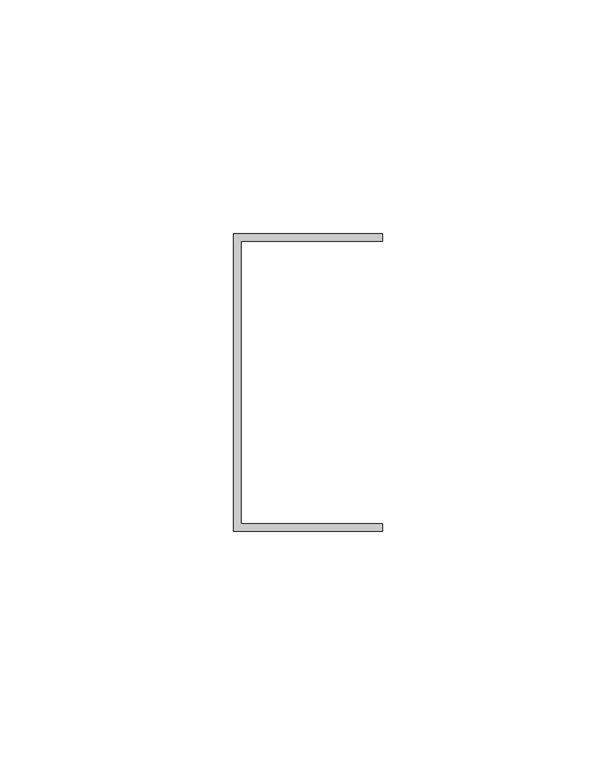
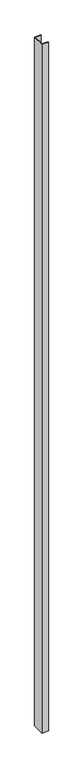
"""IFC4 building model written with IfcOpenShell, lengths in millimetres: proxy geometry, Generic Models 7:Generic Models 1:3:Generic Models 1:3 : Generic Models 7:Generic Models 1:305549:3:Generic Models 1:3:Generic Models 1:3 : Generic Models 7:Generic Models 1:305549:3 : Generic Models 7:Generic Models 1:3:Generic Models 1:3 : Generic Models 7:Generic Models 1:305549:301244:30 : Generic Models 7:Generic Models 1:3:Generic Models 1:3 : Generic Models 7:Generic Models 1:305549:3:Generic Models 1:3:Generic Models 1:3 : Generic Models 7:Generic Models 1:305549:3 : Generic Models 7:Generic Models 1:3:Generic Models 1:3 : Generic Models 7:Generic Models 1:305549:301244:308848."""

from ifc_helpers import new_model, si_unit, frame, origin, place, context, project, spatial, polyline, outline, extrude, source, transform, mapped, element, save


def generic_models_0b7faaaa(model_context):
    return source(origin(), model_context, "Body", "SweptSolid", [
        extrude(outline(polyline([(593738.0867239, -579013.3913841), (593769.8367239, -579013.3913841), (593769.8367239, -579014.9788841), (593739.6742239, -579014.9788841), (593739.6742239, -579075.3038841), (593769.8367239, -579075.3038841), (593769.8367239, -579076.8913841), (593738.0867239, -579076.8913841), (593738.0867239, -579013.3913841)])), frame((0.0, 0.0, 38.1), z_axis=(0.0, 0.0, 1.0), x_axis=(1.0, 0.0, 0.0)), (0.0, 0.0, 1.0), 3657.6),
    ])


if __name__ == "__main__":
    model = new_model("IFC4")
    model_context = context("Model", 3, world=origin())
    ifc_project = project(units=[si_unit("LENGTHUNIT", "METRE", prefix="MILLI")], contexts=[model_context])
    site = spatial("IfcSite", under=ifc_project)
    building = spatial("IfcBuilding", under=site)
    placement = place(None, origin())
    generic_models_shape = generic_models_0b7faaaa(model_context)
    element("IfcBuildingElementProxy", 1, Name="Generic Models 7:Generic Models 1:3:Generic Models 1:3 : Generic Models 7:Generic Models 1:305549:3:Generic Models 1:3:Generic Models 1:3 : Generic Models 7:Generic Models 1:305549:3 : Generic Models 7:Generic Models 1:3:Generic Models 1:3 : Generic Models 7:Generic Models 1:305549:301244:30 : Generic Models 7:Generic Models 1:3:Generic Models 1:3 : Generic Models 7:Generic Models 1:305549:3:Generic Models 1:3:Generic Models 1:3 : Generic Models 7:Generic Models 1:305549:3 : Generic Models 7:Generic Models 1:3:Generic Models 1:3 : Generic Models 7:Generic Models 1:305549:301244:308848", ObjectType="Generic Models 7:Generic Models 1:3:Generic Models 1:3 : Generic Models 7:Generic Models 1:305549:3:Generic Models 1:3:Generic Models 1:3 : Generic Models 7:Generic Models 1:305549:3 : Generic Models 7:Generic Models 1:3:Generic Models 1:3 : Generic Models 7:Generic Models 1:305549:301244:30 : Generic Models 7:Generic Models 1:3:Generic Models 1:3 : Generic Models 7:Generic Models 1:305549:3:Generic Models 1:3:Generic Models 1:3 : Generic Models 7:Generic Models 1:305549:3 : Generic Models 7:Generic Models 1:3:Generic Models 1:3 : Generic Models 7:Generic Models 1:305549:301244:308848", at=placement, inside=building, context=model_context, shape_type="MappedRepresentation", body=[
        mapped(generic_models_shape, transform((0.0, 0.0, 0.0), x_axis=(1.0, 0.0, 0.0), y_axis=(0.0, 1.0, 0.0), z_axis=(0.0, 0.0, 1.0))),
    ])
    save(model, "model.ifc")

# Revit data of these elements
# Type "Generic Models 7:Generic Models 1:3:Generic Models 1:3 : Generic Models 7:Generic Models 1:305549:3:Generic Models 1:3:Generic Models 1:3 : Generic Models 7:Generic Models 1:305549:3 : Generic Models 7:Generic Models 1:3:Generic Models 1:3 : Generic Models 7:Generic Models 1:305549:301244:30 : Generic Models 7:Generic Models 1:3:Generic Models 1:3 : Generic Models 7:Generic Models 1:305549:3:Generic Models 1:3:Generic Models 1:3 : Generic Models 7:Generic Models 1:305549:3 : Generic Models 7:Generic Models 1:3:Generic Models 1:3 : Generic Models 7:Generic Models 1:305549:301244:308848"
#   NameOverride = "Generic Models 7:Generic Models 1:3:Generic Models 1:3 : Generic Models 7:Generic Models 1:305549:3:Generic Models 1:3:Generic Models 1:3 : Generic Models 7:Generic Models 1:305549:3 : Generic Models 7:Generic Models 1:3:Generic Models 1:3 : Generic Models 7:Generic Models 1:305549:301244:308848"
#   ObjectTypeOverride = "Generic Models 1:3:Generic Models 1:3 : Generic Models 7:Generic Models 1:305549:3 : Generic Models 7:Generic Models 1:3:Generic Models 1:3 : Generic Models 7:Generic Models 1:305549:301244"
#   Reference = "Generic Models 1"
#   Tag = "308848"
# Element 1 (IfcBuildingElementProxy, "Generic Models 7:Generic Models 1:3:Generic Models 1:3 : Generic Models 7:Generic Models 1:305549:3:Generic Models 1:3:Generic Models 1:3 : Generic Models 7:Generic Models 1:305549:3 : Generic Models 7:Generic Models 1:3:Generic Models 1:3 : Generic Models 7:Generic Models 1:305549:301244:30 : Generic Models 7:Generic Models 1:3:Generic Models 1:3 : Generic Models 7:Generic Models 1:305549:3:Generic Models 1:3:Generic Models 1:3 : Generic Models 7:Generic Models 1:305549:3 : Generic Models 7:Generic Models 1:3:Generic Models 1:3 : Generic Models 7:Generic Models 1:305549:301244:308848")
#   Materials on its faces: "GALVANIZED U-CHANNEL (250T125-33)"
# Materials
#   "GALVANIZED U-CHANNEL (250T125-33)": class "Unassigned", colour RGB 202 201 200, transparency 0, Keynote = "M05451300.02", Cost = 0
